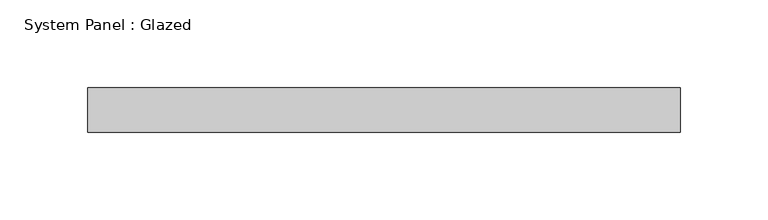
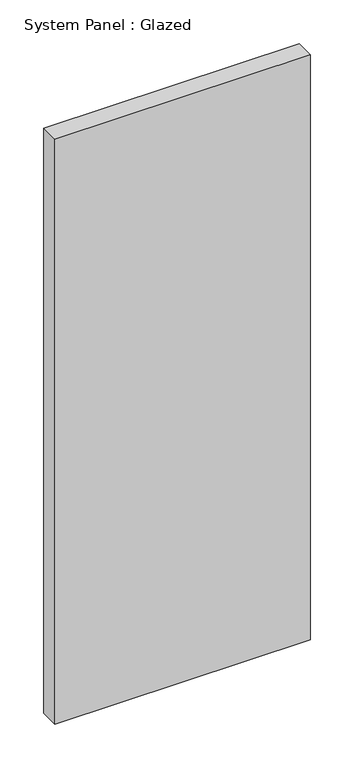
"""IFC4 building model written with IfcOpenShell, lengths in millimetres: plate geometry, System Panel : Glazed."""

from ifc_helpers import new_model, si_unit, origin, origin_with_axes, place, context, project, spatial, polyline, outline, extrude, source, transform, mapped, element, save


def system_panel_glazed_76438ca1(model_context):
    return source(origin(), model_context, "Body", "SweptSolid", [
        extrude(outline(polyline([(169.1789296, 19.05), (-169.1789296, 19.05), (-169.1789296, 44.45), (169.1789296, 44.45), (169.1789296, 19.05)])), origin_with_axes(), (0.0, 0.0, 1.0), 819.15),
    ])


if __name__ == "__main__":
    model = new_model("IFC4")
    model_context = context("Model", 3, world=origin())
    ifc_project = project(units=[si_unit("LENGTHUNIT", "METRE", prefix="MILLI")], contexts=[model_context])
    site = spatial("IfcSite", under=ifc_project)
    building = spatial("IfcBuilding", under=site)
    placement = place(None, origin())
    system_panel_glazed_shape = system_panel_glazed_76438ca1(model_context)
    element("IfcPlate", 1, ObjectType="System Panel : Glazed", at=placement, inside=building, context=model_context, shape_type="MappedRepresentation", body=[
        mapped(system_panel_glazed_shape, transform((0.0, 0.0, 0.0), x_axis=(1.0, 0.0, 0.0), y_axis=(0.0, 1.0, 0.0), z_axis=(0.0, 0.0, 1.0))),
    ])
    save(model, "model.ifc")

# Revit data of these elements
# Element 1 (IfcPlate, "System Panel : Glazed")
#   Materials on its faces: "Glass"
# Materials
#   "Glass": class "Glass", colour RGB 0 128 192, transparency 0.75
